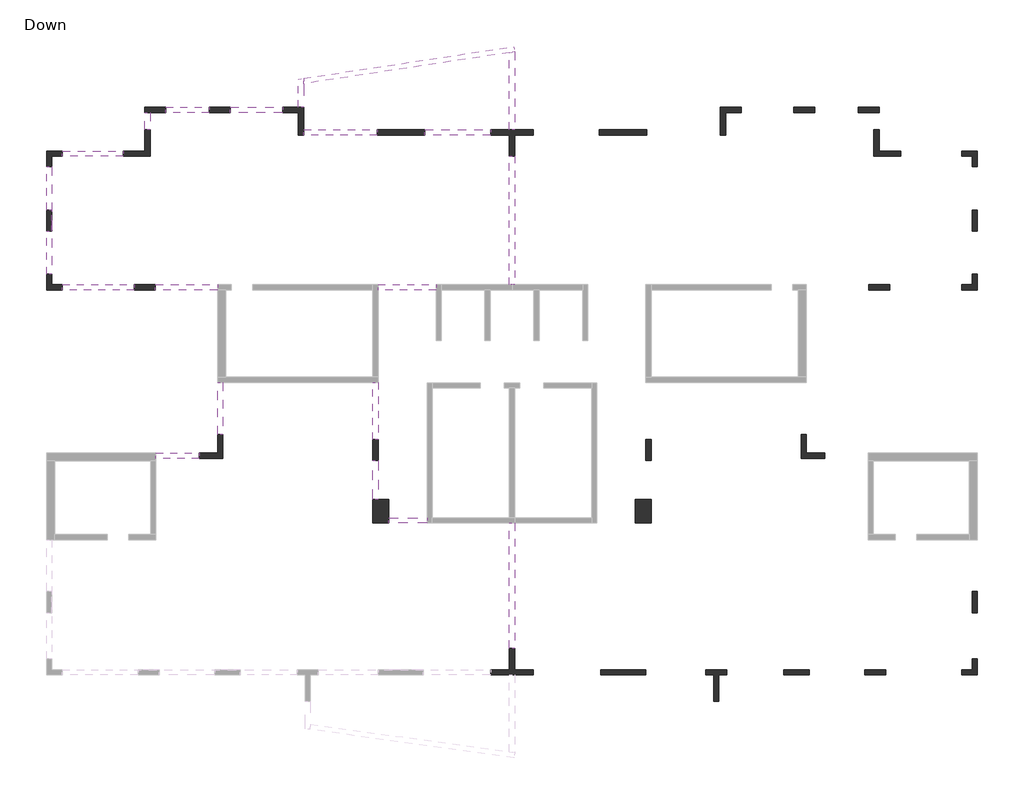
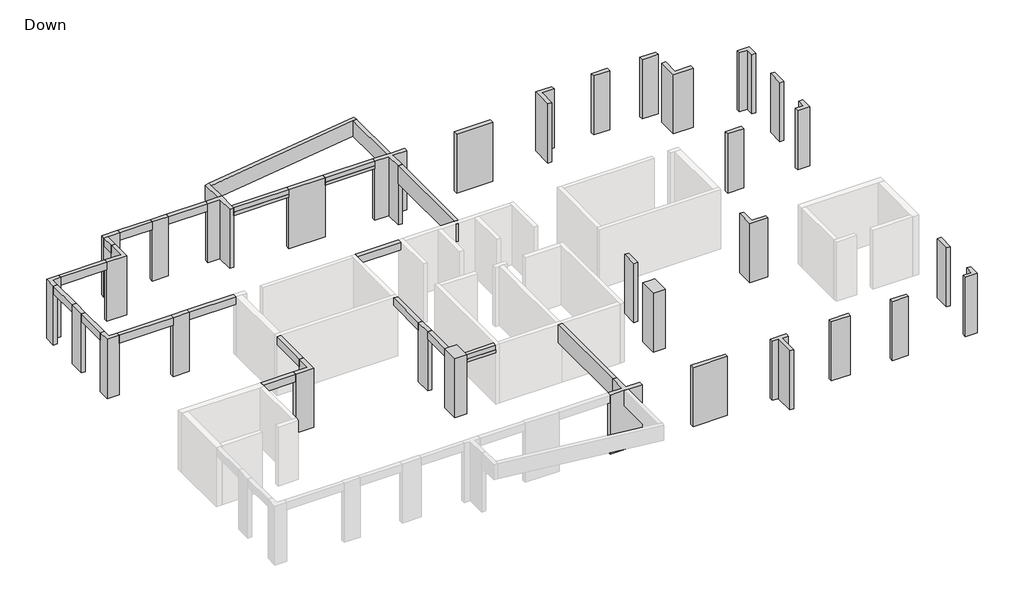
# One storey, part 2 of 2: 32 columns, 21 beams.
# Revit data of these elements (continued)
# Element 26 (IfcColumn, "Concrete Rectengular Column : 80/20")
#   Comments = ""
#   Mark = "C6"
#   SOFiSTiK_AMG_Comments = ""
#   SOFiSTiK_AMG_Scheduled = yes
#   SOFiSTiK_AMG_Adjusted = yes
#   Structural Material = Concrete
#   Phase Created = New Construction
#   Materials on its faces: "Concrete"
# Element 27 (IfcColumn, "Concrete Rectengular Column : 80/20")
#   Comments = ""
#   Mark = "C7"
#   SOFiSTiK_AMG_Comments = ""
#   SOFiSTiK_AMG_Scheduled = yes
#   SOFiSTiK_AMG_Adjusted = yes
#   Structural Material = Concrete
#   Phase Created = New Construction
#   Materials on its faces: "Concrete"
# Element 28 (IfcColumn, "Concrete Rectengular Column : 80/20")
#   Comments = ""
#   Mark = "C9"
#   SOFiSTiK_AMG_Comments = ""
#   SOFiSTiK_AMG_Scheduled = yes
#   SOFiSTiK_AMG_Adjusted = yes
#   Structural Material = Concrete
#   Phase Created = New Construction
#   Materials on its faces: "Concrete"
# Element 29 (IfcColumn, "Concrete Rectengular Column : 80/20")
#   Comments = ""
#   Mark = "C11"
#   SOFiSTiK_AMG_Comments = ""
#   SOFiSTiK_AMG_Scheduled = yes
#   SOFiSTiK_AMG_Adjusted = yes
#   Structural Material = Concrete
#   Phase Created = New Construction
#   Materials on its faces: "Concrete"
# Element 30 (IfcColumn, "Concrete Rectengular Column : 80/20")
#   Comments = ""
#   Mark = "C12"
#   SOFiSTiK_AMG_Comments = ""
#   SOFiSTiK_AMG_Scheduled = yes
#   SOFiSTiK_AMG_Adjusted = yes
#   Structural Material = Concrete
#   Phase Created = New Construction
#   Materials on its faces: "Concrete"
# Element 31 (IfcColumn, "Concrete Rectengular Column : 80/20")
#   Comments = ""
#   Mark = "C13"
#   SOFiSTiK_AMG_Comments = ""
#   SOFiSTiK_AMG_Scheduled = yes
#   SOFiSTiK_AMG_Adjusted = yes
#   Structural Material = Concrete
#   Phase Created = New Construction
#   Materials on its faces: "Concrete"
# Element 32 (IfcColumn, "Concrete Rectengular Column : 80/20")
#   Comments = ""
#   Mark = "C14"
#   SOFiSTiK_AMG_Comments = ""
#   SOFiSTiK_AMG_Scheduled = yes
#   SOFiSTiK_AMG_Adjusted = yes
#   Structural Material = Concrete
#   Phase Created = New Construction
#   Materials on its faces: "Concrete"
# Element 33 (IfcColumn, "Concrete Rectengular Column : 80/20")
#   Comments = ""
#   Mark = "C15"
#   SOFiSTiK_AMG_Comments = ""
#   SOFiSTiK_AMG_Scheduled = yes
#   SOFiSTiK_AMG_Adjusted = yes
#   Structural Material = Concrete
#   Phase Created = New Construction
#   Materials on its faces: "Concrete"
# Element 34 (IfcColumn, "Concrete Rectengular Column : 80/20")
#   Comments = ""
#   Mark = "C16"
#   SOFiSTiK_AMG_Comments = ""
#   SOFiSTiK_AMG_Scheduled = yes
#   SOFiSTiK_AMG_Adjusted = yes
#   Structural Material = Concrete
#   Phase Created = New Construction
#   Materials on its faces: "Concrete"
# Element 35 (IfcColumn, "Concrete Rectengular Column : 80/20")
#   Comments = ""
#   Mark = "C17"
#   SOFiSTiK_AMG_Comments = ""
#   SOFiSTiK_AMG_Scheduled = yes
#   SOFiSTiK_AMG_Adjusted = yes
#   Structural Material = Concrete
#   Phase Created = New Construction
#   Materials on its faces: "Concrete"
# Element 36 (IfcColumn, "Concrete Rectengular Column : 80/20")
#   Comments = ""
#   Mark = "C18"
#   SOFiSTiK_AMG_Comments = ""
#   SOFiSTiK_AMG_Scheduled = yes
#   SOFiSTiK_AMG_Adjusted = yes
#   Structural Material = Concrete
#   Phase Created = New Construction
#   Materials on its faces: "Concrete"
# Element 37 (IfcColumn, "Concrete Rectengular Column : 90/60")
#   Comments = ""
#   Mark = "C19"
#   SOFiSTiK_AMG_Comments = ""
#   SOFiSTiK_AMG_Scheduled = yes
#   SOFiSTiK_AMG_Adjusted = yes
#   Structural Material = Concrete
#   Phase Created = New Construction
#   Materials on its faces: "Concrete"
# Element 38 (IfcColumn, "Concrete Rectengular Column : 90/60")
#   Comments = ""
#   Mark = "C20"
#   SOFiSTiK_AMG_Comments = ""
#   SOFiSTiK_AMG_Scheduled = yes
#   SOFiSTiK_AMG_Adjusted = yes
#   Structural Material = Concrete
#   Phase Created = New Construction
#   Materials on its faces: "Concrete"
# Element 39 (IfcColumn, "Concrete Rectengular Column : 95/20")
#   Comments = ""
#   Mark = "C22"
#   SOFiSTiK_AMG_Comments = ""
#   SOFiSTiK_AMG_Scheduled = yes
#   SOFiSTiK_AMG_Adjusted = yes
#   Structural Material = Concrete
#   Phase Created = New Construction
#   Materials on its faces: "Concrete"
# Element 40 (IfcColumn, "L Column : 100/100/20/20")
#   Comments = ""
#   Mark = "C23"
#   SOFiSTiK_AMG_Comments = ""
#   SOFiSTiK_AMG_Scheduled = yes
#   SOFiSTiK_AMG_Adjusted = yes
#   Structural Material = Concrete
#   Phase Created = New Construction
# Element 41 (IfcColumn, "L Column : 105/80/20/20")
#   Comments = ""
#   Mark = "C25"
#   SOFiSTiK_AMG_Comments = ""
#   SOFiSTiK_AMG_Scheduled = yes
#   SOFiSTiK_AMG_Adjusted = yes
#   Structural Material = Concrete
#   Phase Created = New Construction
# Element 42 (IfcColumn, "L Column : 100/100/20/20")
#   Comments = ""
#   Mark = "C24"
#   SOFiSTiK_AMG_Comments = ""
#   SOFiSTiK_AMG_Scheduled = yes
#   SOFiSTiK_AMG_Adjusted = yes
#   Structural Material = Concrete
#   Phase Created = New Construction
# Element 43 (IfcColumn, "L Column : 105/80/20/20")
#   Comments = ""
#   Mark = "C26"
#   SOFiSTiK_AMG_Comments = ""
#   SOFiSTiK_AMG_Scheduled = yes
#   SOFiSTiK_AMG_Adjusted = yes
#   Structural Material = Concrete
#   Phase Created = New Construction
# Element 44 (IfcColumn, "L Column : 60/60/20/20")
#   Comments = ""
#   Mark = "C27"
#   SOFiSTiK_AMG_Comments = ""
#   SOFiSTiK_AMG_Scheduled = yes
#   SOFiSTiK_AMG_Adjusted = yes
#   Structural Material = Concrete
#   Phase Created = New Construction
# Element 45 (IfcColumn, "L Column : 60/60/20/20")
#   Comments = ""
#   Mark = "C28"
#   SOFiSTiK_AMG_Comments = ""
#   SOFiSTiK_AMG_Scheduled = yes
#   SOFiSTiK_AMG_Adjusted = yes
#   Structural Material = Concrete
#   Phase Created = New Construction
# Element 46 (IfcColumn, "L Column : 60/60/20/20")
#   Comments = ""
#   Mark = "C30"
#   SOFiSTiK_AMG_Comments = ""
#   SOFiSTiK_AMG_Scheduled = yes
#   SOFiSTiK_AMG_Adjusted = yes
#   Structural Material = Concrete
#   Phase Created = New Construction
# Element 47 (IfcColumn, "L Column : 60/60/20/20")
#   Comments = ""
#   Mark = "C31"
#   SOFiSTiK_AMG_Comments = ""
#   SOFiSTiK_AMG_Scheduled = yes
#   SOFiSTiK_AMG_Adjusted = yes
#   Structural Material = Concrete
#   Phase Created = New Construction
# Element 48 (IfcColumn, "L Column : 60/60/20/20")
#   Comments = ""
#   Mark = "C32"
#   SOFiSTiK_AMG_Comments = ""
#   SOFiSTiK_AMG_Scheduled = yes
#   SOFiSTiK_AMG_Adjusted = yes
#   Structural Material = Concrete
#   Phase Created = New Construction
# Element 49 (IfcColumn, "L Column : 90/90/20/20")
#   Comments = ""
#   Mark = "C33"
#   SOFiSTiK_AMG_Comments = ""
#   SOFiSTiK_AMG_Scheduled = yes
#   SOFiSTiK_AMG_Adjusted = yes
#   Structural Material = Concrete
#   Phase Created = New Construction
# Element 50 (IfcColumn, "L Column : 90/90/20/20")
#   Comments = ""
#   Mark = "C34"
#   SOFiSTiK_AMG_Comments = ""
#   SOFiSTiK_AMG_Scheduled = yes
#   SOFiSTiK_AMG_Adjusted = yes
#   Structural Material = Concrete
#   Phase Created = New Construction
# Element 51 (IfcColumn, "T Column : 160/100/20/20")
#   Comments = ""
#   Mark = "C37"
#   SOFiSTiK_AMG_Comments = ""
#   SOFiSTiK_AMG_Scheduled = yes
#   SOFiSTiK_AMG_Adjusted = yes
#   Structural Material = Concrete
#   Phase Created = New Construction
# Element 52 (IfcColumn, "T Column : 160/100/20/20")
#   Comments = ""
#   Mark = "C38"
#   SOFiSTiK_AMG_Comments = ""
#   SOFiSTiK_AMG_Scheduled = yes
#   SOFiSTiK_AMG_Adjusted = yes
#   Structural Material = Concrete
#   Phase Created = New Construction
# Element 53 (IfcColumn, "T Column : 120/80/20/20")
#   Comments = ""
#   Mark = "C36"
#   SOFiSTiK_AMG_Comments = ""
#   SOFiSTiK_AMG_Scheduled = yes
#   SOFiSTiK_AMG_Adjusted = yes
#   Structural Material = Concrete
#   Phase Created = New Construction
# Materials
#   "Concrete": class "Concrete", colour RGB 192 192 192, transparency 0, Keynote = "01000", Description = "Cast-in-place concrete", Cost = 0
#   "Concrete, Cast-in-Place gray": class "Concrete", colour RGB 192 192 192, transparency 0, Description = "Cast-in-place concrete", Cost = 0
